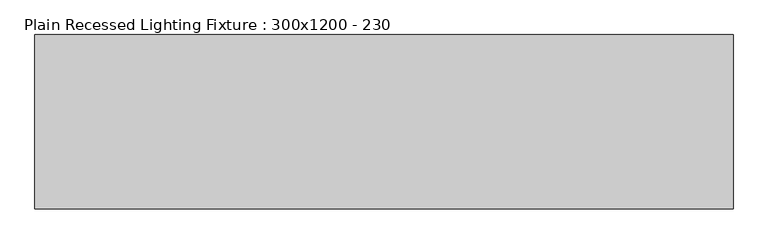
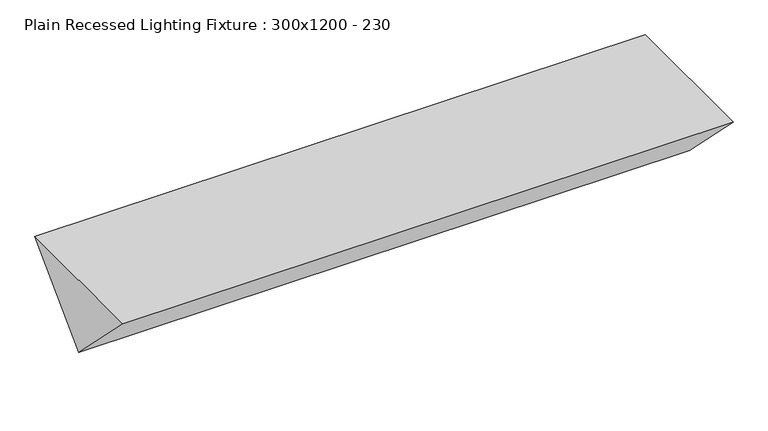
"""IFC4 building model written with IfcOpenShell, lengths in millimetres: light fixture geometry, Plain Recessed Lighting Fixture : 300x1200 - 230."""

import ifcopenshell
import ifcopenshell.guid

model = None  # the IFC model being written
_history = None  # IfcOwnerHistory: only IFC2X3 demands one
_inside = {}  # id of a spatial element -> (the spatial element, [elements in it])
_under = {}  # id of a project, library or spatial element -> (it, [spatial elements below it])
_declared = {}  # id of a project -> (the project, [libraries it declares])
_typed = {}  # id of a type object -> (the type object, [elements of that type])
_made_of = {}  # id of a material, layer set ... -> (it, [elements and type objects made of it])


def new_model(schema):
    """Start an empty IFC model of exactly this schema.

    Asked for "IFC4X3", IfcOpenShell would pick the latest addendum, in which some entities
    have other attributes; the version numbers below select the first issue.
    IFC2X3 requires an IfcOwnerHistory on every rooted entity: one is made here for all.
    """
    global model, _history
    if schema == "IFC4X3":
        model = ifcopenshell.file(schema_version=(4, 3, 0, 0))
    else:
        model = ifcopenshell.file(schema=schema)
    _inside.clear()
    _under.clear()
    _declared.clear()
    _typed.clear()
    _made_of.clear()
    _history = None
    if model.schema == "IFC2X3":
        org = make("IfcOrganization", Name="unknown")
        user = make(
            "IfcPersonAndOrganization",
            ThePerson=make("IfcPerson", FamilyName="unknown"),
            TheOrganization=org,
        )
        app = make(
            "IfcApplication",
            ApplicationDeveloper=org,
            Version="unknown",
            ApplicationFullName="unknown",
            ApplicationIdentifier="unknown",
        )
        _history = make(
            "IfcOwnerHistory",
            OwningUser=user,
            OwningApplication=app,
            ChangeAction="ADDED",
            CreationDate=0,
        )
    return model


def make(cls, **values):
    """One entity of the class cls with the attributes given. An attribute that is None is left unset."""
    return model.create_entity(
        cls, **{name: value for name, value in values.items() if value is not None}
    )


def rooted(cls, **values):
    """An entity with a GlobalId (a new one), such as an element, a storey or a relation."""
    return make(cls, GlobalId=ifcopenshell.guid.new(), OwnerHistory=_history, **values)


def si_unit(unit_type, name, prefix=None):
    """IfcSIUnit, for example si_unit("LENGTHUNIT", "METRE", prefix="MILLI")."""
    return make("IfcSIUnit", UnitType=unit_type, Prefix=prefix, Name=name)


def assignment(units):
    """IfcUnitAssignment: the units of a project."""
    return None if units is None else make("IfcUnitAssignment", Units=units)


def point(xyz):
    """IfcCartesianPoint."""
    return None if xyz is None else make("IfcCartesianPoint", Coordinates=xyz)


def direction(xyz):
    """IfcDirection."""
    return None if xyz is None else make("IfcDirection", DirectionRatios=xyz)


def frame(location, z_axis=None, x_axis=None):
    """IfcAxis2Placement3D, a coordinate frame: its origin and axes. An axis left out is left unset."""
    return make(
        "IfcAxis2Placement3D",
        Location=point(location),
        Axis=direction(z_axis),
        RefDirection=direction(x_axis),
    )


def origin():
    """The frame at (0, 0, 0) with its axes left unset."""
    return frame((0.0, 0.0, 0.0))


def place(relative_to, where):
    """IfcLocalPlacement: puts the frame where relative to a parent placement (None: the world)."""
    return make(
        "IfcLocalPlacement", PlacementRelTo=relative_to, RelativePlacement=where
    )


def context(
    kind, dimensions, precision=None, world=None, true_north=None, identifier=None
):
    """IfcGeometricRepresentationContext, for example the 3D "Model" context."""
    return make(
        "IfcGeometricRepresentationContext",
        ContextIdentifier=identifier,
        ContextType=kind,
        CoordinateSpaceDimension=dimensions,
        Precision=precision,
        WorldCoordinateSystem=world,
        TrueNorth=true_north,
    )


def project(units=None, contexts=None):
    """IfcProject with its units and contexts."""
    return rooted(
        "IfcProject",
        Name="project",
        RepresentationContexts=contexts,
        UnitsInContext=assignment(units),
    )


def spatial(cls, under=None, at=None, **own):
    """A site, building, storey or space (cls), placed at a placement, below another one or the project."""
    s = rooted(cls, ObjectPlacement=at, **own)
    if under is not None:
        _under.setdefault(under.id(), (under, []))[1].append(s)
    return s


def polyline(points):
    """IfcPolyline through the points."""
    return make("IfcPolyline", Points=[point(p) for p in points])


def outline(outer, holes=None, kind="AREA"):
    """IfcArbitraryClosedProfileDef: a profile drawn as a closed curve; with holes, ...WithVoids."""
    if holes is None:
        return make("IfcArbitraryClosedProfileDef", ProfileType=kind, OuterCurve=outer)
    return make(
        "IfcArbitraryProfileDefWithVoids",
        ProfileType=kind,
        OuterCurve=outer,
        InnerCurves=holes,
    )


def extrude(swept, where, along, depth):
    """IfcExtrudedAreaSolid: the profile swept, set in the frame where, extruded along a direction by depth."""
    return make(
        "IfcExtrudedAreaSolid",
        SweptArea=swept,
        Position=where,
        ExtrudedDirection=direction(along),
        Depth=depth,
    )


def shape(context_of_items, identifier, shape_type, items):
    """IfcShapeRepresentation: the items that make up one representation, for example the "Body"."""
    return make(
        "IfcShapeRepresentation",
        ContextOfItems=context_of_items,
        RepresentationIdentifier=identifier,
        RepresentationType=shape_type,
        Items=items,
    )


def source(mapping_origin, context_of_items, identifier, shape_type, items):
    """IfcRepresentationMap: a shape defined once, which mapped items show again and again."""
    return make(
        "IfcRepresentationMap",
        MappingOrigin=mapping_origin,
        MappedRepresentation=shape(context_of_items, identifier, shape_type, items),
    )


def transform(
    local_origin,
    x_axis=None,
    y_axis=None,
    z_axis=None,
    scale=None,
    scale2=None,
    scale3=None,
    uniform=True,
):
    """IfcCartesianTransformationOperator3D, or its non-uniform kind. x_axis, y_axis, z_axis: its Axis1, 2, 3."""
    if uniform:
        return make(
            "IfcCartesianTransformationOperator3D",
            Axis1=direction(x_axis),
            Axis2=direction(y_axis),
            LocalOrigin=point(local_origin),
            Scale=scale,
            Axis3=direction(z_axis),
        )
    return make(
        "IfcCartesianTransformationOperator3DnonUniform",
        Axis1=direction(x_axis),
        Axis2=direction(y_axis),
        LocalOrigin=point(local_origin),
        Scale=scale,
        Axis3=direction(z_axis),
        Scale2=scale2,
        Scale3=scale3,
    )


def mapped(mapping_source, mapping_target):
    """IfcMappedItem: shows the shape of a source again, moved by a transform."""
    return make(
        "IfcMappedItem", MappingSource=mapping_source, MappingTarget=mapping_target
    )


def made_of(thing, what):
    """Note that an element or type object is made of a material, layer set ...; save() writes the relation."""
    if what is not None:
        _made_of.setdefault(what.id(), (what, []))[1].append(thing)
    return thing


def element(
    cls,
    number,
    at=None,
    inside=None,
    cuts=None,
    type_object=None,
    material=None,
    context=None,
    identifier="Body",
    shape_type=None,
    held_by="IfcProductDefinitionShape",
    body=None,
    shapes=None,
    **own,
):
    """One element of the class cls, such as IfcWall. Its Tag is "e" and its number.

    at: its placement. inside: the storey or other place that contains it. cuts: it is an
    opening in that element (IfcRelVoidsElement). A single representation is given by context,
    identifier, shape_type and body (its items); several are given by shapes. held_by: the class
    of the entity that holds the representations. save() writes the other relations.
    """
    e = rooted(cls, Tag="e%d" % number, ObjectPlacement=at, **own)
    if body is not None:
        shapes = [shape(context, identifier, shape_type, body)]
    if shapes is not None:
        e.Representation = make(held_by, Representations=shapes)
    if inside is not None:
        _inside.setdefault(inside.id(), (inside, []))[1].append(e)
    if cuts is not None:
        rooted(
            "IfcRelVoidsElement", RelatingBuildingElement=cuts, RelatedOpeningElement=e
        )
    if type_object is not None:
        _typed.setdefault(type_object.id(), (type_object, []))[1].append(e)
    return made_of(e, material)


def aggregate(whole, parts):
    """IfcRelAggregates: a whole, such as a stair, and the parts it consists of."""
    return rooted("IfcRelAggregates", RelatingObject=whole, RelatedObjects=parts)


def save(model, path):
    """Write the relations noted so far, then the file.

    IfcRelAggregates (storeys below a building ...), IfcRelContainedInSpatialStructure (elements
    in a storey), IfcRelDefinesByType, IfcRelAssociatesMaterial and IfcRelDeclares: one each for
    every whole, place, type object, material and project.
    """
    for whole, parts in _under.values():
        aggregate(whole, parts)
    for where, things in _inside.values():
        rooted(
            "IfcRelContainedInSpatialStructure",
            RelatedElements=things,
            RelatingStructure=where,
        )
    for kind, things in _typed.values():
        rooted("IfcRelDefinesByType", RelatedObjects=things, RelatingType=kind)
    for what, things in _made_of.values():
        rooted("IfcRelAssociatesMaterial", RelatedObjects=things, RelatingMaterial=what)
    for by, libraries in _declared.values():
        rooted("IfcRelDeclares", RelatingContext=by, RelatedDefinitions=libraries)
    model.write(path)


def plain_recessed_lighting_fixture_300x1200_230_e46e8774(model_context):
    return source(origin(), model_context, "Body", "SweptSolid", [
        extrude(outline(polyline([(-300.0, 0.0), (0.0, 0.0), (-150.0, -150.0), (-300.0, 0.0)])), frame((0.0, 0.0, 0.0), z_axis=(1.0, 0.0, 0.0), x_axis=(0.0, 1.0, 0.0)), (0.0, 0.0, 1.0), 1200.0),
    ])


if __name__ == "__main__":
    model = new_model("IFC4")
    model_context = context("Model", 3, world=origin())
    ifc_project = project(units=[si_unit("LENGTHUNIT", "METRE", prefix="MILLI")], contexts=[model_context])
    site = spatial("IfcSite", under=ifc_project)
    building = spatial("IfcBuilding", under=site)
    placement = place(None, origin())
    plain_recessed_lighting_fixture_300x1200_230_shape = plain_recessed_lighting_fixture_300x1200_230_e46e8774(model_context)
    element("IfcLightFixture", 1, ObjectType="Plain Recessed Lighting Fixture : 300x1200 - 230", at=placement, inside=building, context=model_context, shape_type="MappedRepresentation", body=[
        mapped(plain_recessed_lighting_fixture_300x1200_230_shape, transform((0.0, 0.0, 0.0), x_axis=(1.0, 0.0, 0.0), y_axis=(0.0, 1.0, 0.0), z_axis=(0.0, 0.0, 1.0))),
    ])
    save(model, "model.ifc")

# Revit data of these elements
# Type "Plain Recessed Lighting Fixture : 300x1200 - 230"
#   Photometric Web File = "1x42A12.ies"
#   Width = 300 mm
#   Wattage = 64 W
#   built-in parameter 1150110 = 1 (stored number, unit not read)
#   built-in parameter 1150109 = 1 (stored number, unit not read)
#   built-in parameter 1150113 = 1 (stored number, unit not read)
#   Tilt Angle = -90.00°
#   Lumens = 5699.84 lm
#   built-in parameter 1114217 = 0.88 (stored number, unit not read)
#   built-in parameter 1150115 = 1 (stored number, unit not read)
#   built-in parameter 1150105 = 453.579 (stored number, unit not read)
#   Length = 1200 mm
#   built-in parameter 1150112 = 1 (stored number, unit not read)
#   built-in parameter 1150114 = 1 (stored number, unit not read)
#   built-in parameter 1150107 = 4230 (stored number, unit not read)
#   built-in parameter 1150106 = 4.53579 (stored number, unit not read)
#   Emit from Rectangle Width = 300 mm
#   Emit from Rectangle Length = 1200 mm
#   built-in parameter 1150104 = 8.27394 (stored number, unit not read)
#   Depth = 150 mm
#   Default Elevation = 2000 mm
#   Ballast Voltage = 230 V
#   built-in parameter 1114218 = 0.88 (stored number, unit not read)
#   built-in parameter 1150133 = 10 (stored number, unit not read)
#   Apparent Load = 64 VA
#   built-in parameter 1150134 = 8
#   built-in parameter 1150137 = 1
#   Color Filter = 16777215
#   built-in parameter 1140040 [instance default] = 1
#   Load Classification = Lighting - Dwelling Unit
#   Emit Shape Visible in Rendering = no
#   Dimming Lamp Color Temperature Shift = (empty or 0)
#   Assembly Code = ""
